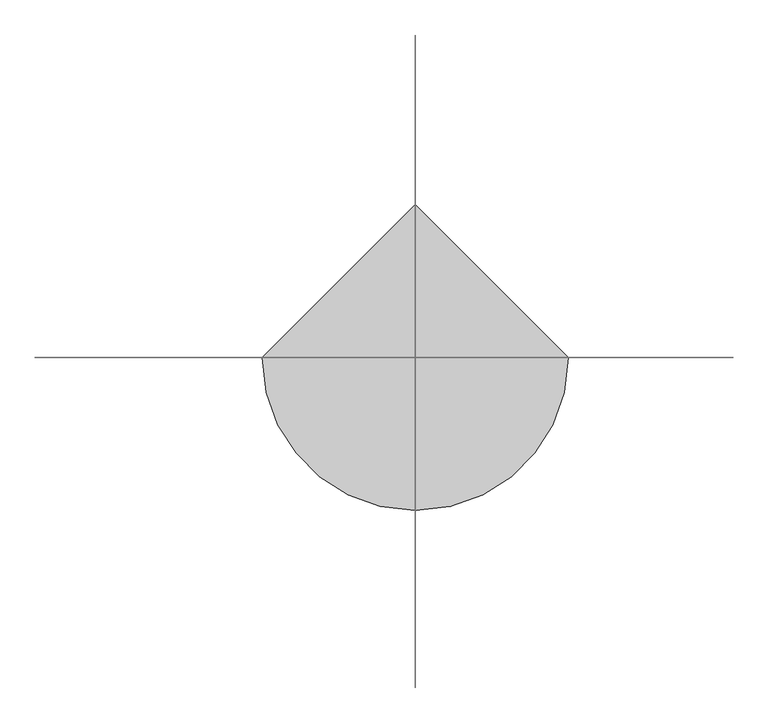
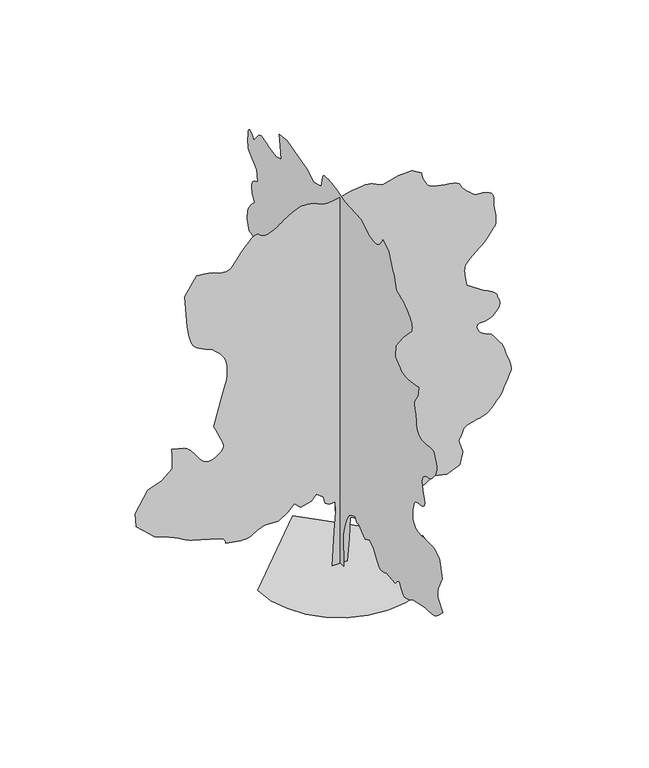
"""IFC4 building model written with IfcOpenShell, lengths in millimetres: geographic element geometry, RPC 木 - 落葉樹 : シュマード オーク - 9.1 メートル."""

from ifc_helpers import new_model, si_unit, origin, place, context, project, spatial, triangles, source, transform, mapped, element, save


def geographic_element_5c09a096(model_context):
    return source(origin(), model_context, "Body", "Tessellation", [
        triangles([(-0.0016876, 163.832478, 0.0085608), (-0.0016876, -150.8808976, 0.0085608), (-0.0016876, -123.5141451, 779.9515205), (-0.0016876, -178.2471505, 1012.5653744), (-0.0016876, -260.3461545, 1231.4963425), (-0.0016876, -356.128771, 1382.0105564), (-0.0016876, -465.5942914, 1450.4274559), (-0.0016876, -602.4255469, 1505.1588535), (-0.0016876, -657.1595243, 1382.0105564), (-0.0016876, -752.9421953, 1409.3763279), (-0.0016876, -862.4076794, 1299.9107712), (-0.0016876, -1012.9218206, 1204.1281002), (-0.0016876, -1190.8042042, 1286.2278854), (-0.0016876, -1355.0011585, 1176.7624014), (-0.0016876, -1464.4667152, 985.1971321), (-0.0016876, -1490.95536, 947.379019), (-0.0016876, -1518.0429508, 911.3556364), (-0.0016876, -1546.3262535, 878.9241858), (-0.0016876, -1576.4068302, 851.8769268), (-0.0016876, -1608.8788307, 832.0111336), (-0.0016876, -1644.3435265, 821.1189205), (-0.0016876, -1683.3976833, 821.0001051), (-0.0016876, -1720.8568794, 827.6608177), (-0.0016876, -1751.8549873, 835.7598146), (-0.0016876, -1777.4640347, 845.0544508), (-0.0016876, -1798.7681122, 855.307168), (-0.0016876, -1816.8392475, 866.2777193), (-0.0016876, -1832.7565899, 877.7285465), (-0.0016876, -1847.5972538, 889.4144611), (-0.0016876, -2203.3595501, 848.3658766), (-0.0016876, -2238.4248516, 888.8583904), (-0.0016876, -2272.772319, 925.9965305), (-0.0016876, -2305.6839729, 956.4360243), (-0.0016876, -2336.4419792, 976.8200272), (-0.0016876, -2364.326033, 983.8017958), (-0.0016876, -2388.6204803, 974.0293545), (-0.0016876, -2408.6076324, 944.1484749), (-0.0016876, -2428.6731228, 901.1838009), (-0.0016876, -2453.5264023, 856.783386), (-0.0016876, -2482.9269333, 814.5366188), (-0.0016876, -2516.6373756, 778.0354311), (-0.0016876, -2554.4225693, 750.8694294), (-0.0016876, -2596.0299133, 736.6279295), (-0.0016876, -2641.2265732, 738.9003925), (-0.0016876, -2686.5496788, 752.2242886), (-0.0016876, -2728.9909836, 768.4198116), (-0.0016876, -2769.0309814, 787.0116274), (-0.0016876, -2807.1751648, 807.5169165), (-0.0016876, -2843.8787384, 829.4580917), (-0.0016876, -2879.6216148, 852.3547319), (-0.0016876, -2914.8839973, 875.7316481), (-0.0016876, -3407.4725349, 971.5142464), (-0.0016876, -3468.9228539, 971.6356052), (-0.0016876, -3529.5136322, 972.4722548), (-0.0016876, -3588.4361984, 974.7472612), (-0.0016876, -3644.831012, 979.1734446), (-0.0016876, -3697.8891106, 986.4761965), (-0.0016876, -3746.7762428, 997.3658661), (-0.0016876, -3790.6081604, 1012.5653744), (-0.0016876, -3832.8471519, 1034.5444107), (-0.0016876, -3877.2604294, 1064.4252903), (-0.0016876, -3923.4427849, 1100.8885443), (-0.0016876, -3971.0916206, 1142.6146311), (-0.0016876, -4019.8017288, 1188.2915668), (-0.0016876, -4069.2199333, 1236.6025715), (-0.0016876, -4119.0171844, 1286.2278854), (-0.0016876, -3927.4367271, 1505.1588535), (-0.0016876, -3921.7492836, 1546.169577), (-0.0016876, -3916.9969574, 1586.9401989), (-0.0016876, -3914.1660255, 1627.2304722), (-0.0016876, -3914.1913147, 1666.8053822), (-0.0016876, -3918.0588112, 1705.4197403), (-0.0016876, -3926.7289215, 1742.8410027), (-0.0016876, -3941.1373444, 1778.8239807), (-0.0016876, -4091.6412392, 2093.5376198), (-0.0016876, -3995.8636551, 2476.6656876), (-0.0016876, -3988.3562645, 2487.2368446), (-0.0016876, -3966.0105354, 2514.3244354), (-0.0016876, -3929.0799408, 2550.9846977), (-0.0016876, -3877.7659218, 2590.2918915), (-0.0016876, -3812.3469498, 2625.276384), (-0.0016876, -3733.0506271, 2649.0121445), (-0.0016876, -3640.1039749, 2654.5478531), (-0.0016876, -3536.5408195, 2650.2507317), (-0.0016876, -3429.8685516, 2648.5572304), (-0.0016876, -3327.0132019, 2648.8098312), (-0.0016876, -3234.9513794, 2650.2507317), (-0.0016876, -3160.5841164, 2652.1465462), (-0.0016876, -3110.8880219, 2653.8400475), (-0.0016876, -3092.7638374, 2654.5478531), (-0.0016876, -3082.1470436, 2661.7773537), (-0.0016876, -3054.7966782, 2682.1514008), (-0.0016876, -3017.3603004, 2713.7991783), (-0.0016876, -2976.5872078, 2754.7490044), (-0.0016876, -2939.1758286, 2803.1562241), (-0.0016876, -2911.8254631, 2857.0482834), (-0.0016876, -2901.2086693, 2914.5302399), (-0.0016876, -2903.2056404, 2971.9613274), (-0.0016876, -2908.7919273, 3027.268998), (-0.0016876, -2917.3611717, 3080.7570122), (-0.0016876, -2928.331723, 3132.8291245), (-0.0016876, -2941.0969322, 3183.8143845), (-0.0016876, -2955.050441, 3234.0668404), (-0.0016876, -2969.6103081, 3283.9652481), (-0.0016876, -2981.5921349, 3298.5756935), (-0.0016876, -2994.9892822, 3312.8070923), (-0.0016876, -3011.2682304, 3326.3306854), (-0.0016876, -3031.8443001, 3338.7927155), (-0.0016876, -3058.1839714, 3349.7885559), (-0.0016876, -3091.7022743, 3359.0150276), (-0.0016876, -3133.8151108, 3366.0675041), (-0.0016876, -3184.7497925, 3370.3899147), (-0.0016876, -3239.7795731, 3375.4201309), (-0.0016876, -3292.8629608, 3386.8964653), (-0.0016876, -3338.0596207, 3410.5816475), (-0.0016876, -3369.3789299, 3452.2395699), (-0.0016876, -3380.8296844, 3517.5826744), (-0.0016876, -3366.4212616, 3612.3742722), (-0.0016876, -3336.9474792, 3719.5267433), (-0.0016876, -3309.8750038, 3817.8070816), (-0.0016876, -3289.2480652, 3906.78479), (-0.0016876, -3279.1370544, 3985.9296684), (-0.0016876, -3283.6617783, 4054.7862213), (-0.0016876, -3306.841468, 4112.8745361), (-0.0016876, -3352.7459335, 4159.6891205), (-0.0016876, -3409.0395905, 4192.4996178), (-0.0016876, -3461.2637283, 4212.5954842), (-0.0016876, -3510.3531738, 4225.7653198), (-0.0016876, -3557.3192024, 4237.7218575), (-0.0016876, -3603.071933, 4254.2534065), (-0.0016876, -3648.5973518, 4281.0479919), (-0.0016876, -3694.8305763, 4323.8936325), (-0.0016876, -3741.9483398, 4378.3926315), (-0.0016876, -3786.8921082, 4436.4809464), (-0.0016876, -3825.8705429, 4498.38647), (-0.0016876, -3855.0411461, 4564.3615128), (-0.0016876, -3870.5617104, 4634.6589661), (-0.0016876, -3868.5900284, 4709.5064323), (-0.0016876, -3845.3344711, 4789.131514), (-0.0016876, -3817.2507202, 4864.434185), (-0.0016876, -3798.2672859, 4925.8842133), (-0.0016876, -3780.7244614, 4972.9516891), (-0.0016876, -3756.9381226, 5005.1811172), (-0.0016876, -3719.2741425, 5022.091713), (-0.0016876, -3660.0733955, 5023.2038544), (-0.0016876, -3571.677047, 5008.0623367), (-0.0016876, -3466.799437, 4991.303476), (-0.0016876, -3365.9916367, 4987.9414719), (-0.0016876, -3273.3231651, 4998.0019043), (-0.0016876, -3192.8638321, 5021.4597748), (-0.0016876, -3128.6584488, 5058.3150833), (-0.0016876, -3084.8265312, 5108.592247), (-0.0016876, -3065.3878922, 5172.2418503), (-0.0016876, -3058.7400421, 5240.239444), (-0.0016876, -3050.651001, 5303.8884659), (-0.0016876, -3041.3489525, 5363.9737518), (-0.0016876, -3031.0859161, 5421.1778183), (-0.0016876, -3020.1153648, 5476.2325974), (-0.0016876, -3008.6646103, 5529.8467667), (-0.0016876, -2996.9862534, 5582.753421), (-0.0016876, -2985.6113663, 5620.8976044), (-0.0016876, -2976.4101837, 5659.1429443), (-0.0016876, -2971.4811241, 5697.6411758), (-0.0016876, -2973.0481796, 5736.4928741), (-0.0016876, -2983.2097687, 5775.8253571), (-0.0016876, -3004.1651756, 5815.7641983), (-0.0016876, -3038.0375267, 5856.4105545), (-0.0016876, -3074.2606064, 5906.2836731), (-0.0016876, -3101.6109718, 5968.8211349), (-0.0016876, -3121.3277916, 6036.6414139), (-0.0016876, -3134.573204, 6102.3129868), (-0.0016876, -3142.5610886, 6158.4049118), (-0.0016876, -3146.4538742, 6197.4839218), (-0.0016876, -3147.4904388, 6212.1702347), (-0.0016876, -3127.318705, 6207.6710907), (-0.0016876, -3073.1481743, 6196.2200455), (-0.0016876, -2994.5596573, 6180.9523727), (-0.0016876, -2901.1328018, 6164.9516052), (-0.0016876, -2802.4231293, 6151.3518539), (-0.0016876, -2708.0358673, 6143.2378143), (-0.0016876, -2627.525956, 6143.7685959), (-0.0016876, -2559.5539421, 6155.5986877), (-0.0016876, -2495.8918396, 6178.2223068), (-0.0016876, -2435.8141113, 6209.8197968), (-0.0016876, -2378.6078648, 6248.5959183), (-0.0016876, -2323.5554111, 6292.7560135), (-0.0016876, -2269.9412418, 6340.5060059), (-0.0016876, -2217.0422905, 6390.0506561), (-0.0016876, -2230.7251762, 6677.4081161), (-0.0016876, -2531.7483719, 7060.5440323), (-0.0016876, -2873.832724, 7416.3037125), (-0.0016876, -2879.1916992, 7460.4132294), (-0.0016876, -2881.4162727, 7505.3825775), (-0.0016876, -2877.4223305, 7552.0204285), (-0.0016876, -2864.1007599, 7601.1604523), (-0.0016876, -2838.3427391, 7653.6624802), (-0.0016876, -2797.0135757, 7710.3351837), (-0.0016876, -2737.0041573, 7772.0633926), (-0.0016876, -2666.6308365, 7831.3905853), (-0.0016876, -2596.257225, 7881.3648605), (-0.0016876, -2525.8914619, 7923.5785629), (-0.0016876, -2455.5207573, 7959.5490417), (-0.0016876, -2385.149762, 7990.8680603), (-0.0016876, -2314.778912, 8019.0779663), (-0.0016876, -2244.408062, 8045.7211075), (-0.0016876, -2223.8648392, 8115.8918243), (-0.0016876, -2203.2002575, 8184.8754044), (-0.0016876, -2182.2954288, 8251.4568054), (-0.0016876, -2161.0317558, 8314.4488907), (-0.0016876, -2139.2903503, 8372.6383621), (-0.0016876, -2116.9523243, 8424.8625), (-0.0016876, -2093.8939934, 8469.9074249), (-0.0016876, -2068.3230251, 8519.0224503), (-0.0016876, -2040.1180607, 8579.6135193), (-0.0016876, -2011.6754654, 8644.7543106), (-0.0016876, -1985.3865177, 8707.4935043), (-0.0016876, -1963.6451122, 8760.9309402), (-0.0016876, -1948.8448528, 8798.0641388), (-0.0016876, -1943.3773087, 8811.991777), (-0.0016876, -1710.7634548, 8948.8206345), (-0.0016876, -1698.8374386, 8925.2366089), (-0.0016876, -1685.7130943, 8900.944487), (-0.0016876, -1670.1925301, 8875.2117554), (-0.0016876, -1651.0851208, 8847.3303177), (-0.0016876, -1627.1900677, 8816.5670792), (-0.0016876, -1597.3090427, 8782.2145248), (-0.0016876, -1560.2493862, 8743.5651398), (-0.0016876, -1515.6087971, 8710.0974152), (-0.0016876, -1464.5071198, 8690.2794388), (-0.0016876, -1408.0188526, 8681.811351), (-0.0016876, -1347.2231449, 8682.4432892), (-0.0016876, -1283.194495, 8689.9003922), (-0.0016876, -1217.0121975, 8701.9072174), (-0.0016876, -1149.7530762, 8716.1894852), (-0.0016876, -848.7223228, 8921.4449799), (-0.0016876, -191.9302724, 8962.4959625), (-0.0016876, -107.0787747, 8985.8276779), (-0.0016876, -23.3040577, 9008.451297), (-0.0016876, 58.316385, 9029.633725), (-0.0016876, 136.7053639, 9048.6680283), (-0.0016876, 210.7859892, 9064.8205307), (-0.0016876, 279.4814509, 9077.3837173), (-0.0016876, 341.7128632, 9085.6494919), (-0.0016876, 403.0696558, 9091.9438751), (-0.0016876, 467.2954957, 9097.530162), (-0.0016876, 530.565798, 9100.0073364), (-0.0016876, 589.0485291, 9096.9738007), (-0.0016876, 638.9140537, 9086.0541183), (-0.0016876, 676.3327726, 9064.8205307), (-0.0016876, 697.4776302, 9030.9231812), (-0.0016876, 765.8919863, 8757.2404678), (-0.0016876, 1066.9227396, 8675.163501), (-0.0016876, 1340.5877941, 8839.3424332), (-0.0016876, 1682.6672047, 8921.4449799), (-0.0016876, 2134.2120266, 9058.2738373), (-0.0016876, 2435.2427799, 9017.2222733), (-0.0016876, 2407.8745377, 8757.2404678), (-0.0016876, 2353.14314, 8456.2320969), (-0.0016876, 2572.0665504, 8387.8054596), (-0.0016876, 2790.9973732, 8428.8564423), (-0.0016876, 2875.6529617, 8460.6556641), (-0.0016876, 2958.0331078, 8489.7004028), (-0.0016876, 3035.8635315, 8513.2338501), (-0.0016876, 3106.8687904, 8528.5015228), (-0.0016876, 3168.7996033, 8532.7733551), (-0.0016876, 3219.3296585, 8523.2692841), (-0.0016876, 3256.2352547, 8497.2580811), (-0.0016876, 3461.49104, 8250.9766022), (-0.0016876, 3508.1286003, 8305.5005997), (-0.0016876, 3553.0726593, 8352.972702), (-0.0016876, 3594.6797127, 8386.33927), (-0.0016876, 3631.2568405, 8398.4978302), (-0.0016876, 3661.1352493, 8382.4209045), (-0.0016876, 3682.6464363, 8331.0315994), (-0.0016876, 3694.0974815, 8237.2762756), (-0.0016876, 3697.5603516, 8133.1570496), (-0.0016876, 3696.7263908, 8052.7480042), (-0.0016876, 3692.302533, 7992.0563599), (-0.0016876, 3684.9974556, 7947.1881683), (-0.0016876, 3675.5433815, 7914.1500687), (-0.0016876, 3664.6486977, 7889.0236954), (-0.0016876, 3653.0462082, 7867.8412674), (-0.0016876, 3338.3378014, 7607.8588806), (-0.0016876, 3310.9618561, 7320.5264191), (-0.0016876, 3354.7176155, 7302.679834), (-0.0016876, 3397.1845001, 7283.418219), (-0.0016876, 3436.9968956, 7261.2748032), (-0.0016876, 3472.8409286, 7234.8345566), (-0.0016876, 3503.4521416, 7202.6307083), (-0.0016876, 3527.4660828, 7163.2476471), (-0.0016876, 3543.5680069, 7115.270343), (-0.0016876, 3549.7359444, 7062.4904251), (-0.0016876, 3545.8178696, 7009.7105072), (-0.0016876, 3533.5328636, 6956.9300079), (-0.0016876, 3514.5491386, 6904.15009), (-0.0016876, 3490.5351974, 6851.3701721), (-0.0016876, 3463.1595428, 6798.5902542), (-0.0016876, 3434.1153854, 6745.8103363), (-0.0016876, 3477.9217232, 6701.8269745), (-0.0016876, 3520.6412086, 6657.6918777), (-0.0016876, 3561.2119881, 6613.3294693), (-0.0016876, 3598.5472092, 6568.6130127), (-0.0016876, 3631.5853088, 6523.4157715), (-0.0016876, 3659.2394348, 6477.6127533), (-0.0016876, 3680.4221535, 6431.1016388), (-0.0016876, 3695.6139587, 6385.7782425), (-0.0016876, 3706.5089333, 6343.3372284), (-0.0016876, 3713.8140106, 6303.2972305), (-0.0016876, 3718.2375778, 6265.1530472), (-0.0016876, 3720.5127296, 6228.4494736), (-0.0016876, 3721.346981, 6192.7068878), (-0.0016876, 3721.4731361, 6157.443924), (-0.0016876, 3639.3708801, 5924.8377731), (-0.0016876, 3601.2772751, 5918.7207047), (-0.0016876, 3563.2848267, 5911.1880249), (-0.0016876, 3525.5449791, 5900.7735443), (-0.0016876, 3488.1591797, 5886.0616516), (-0.0016876, 3451.2788727, 5865.5867386), (-0.0016876, 3414.9546364, 5837.9326126), (-0.0016876, 3379.388784, 5801.6842438), (-0.0016876, 3346.9826225, 5758.63629), (-0.0016876, 3319.6319664, 5711.9990204), (-0.0016876, 3296.4522766, 5662.378212), (-0.0016876, 3276.6093018, 5610.3569687), (-0.0016876, 3259.2940796, 5556.5404861), (-0.0016876, 3243.6723587, 5501.535704), (-0.0016876, 3228.8596001, 5445.9245636), (-0.0016876, 3196.8324852, 5401.9162033), (-0.0016876, 3166.1201157, 5357.806105), (-0.0016876, 3138.0363647, 5313.4436966), (-0.0016876, 3113.8959778, 5268.7022415), (-0.0016876, 3095.0389893, 5223.5050003), (-0.0016876, 3082.7286942, 5177.7269806), (-0.0016876, 3078.3554146, 5131.2158661), (-0.0016876, 3092.0307426, 4761.7558594), (-0.0016876, 3124.0578575, 4758.5203011), (-0.0016876, 3154.7955162, 4753.4897942), (-0.0016876, 3182.8792671, 4744.8955513), (-0.0016876, 3206.9943649, 4730.8914642), (-0.0016876, 3225.8766426, 4709.7087456), (-0.0016876, 3238.1616486, 4679.5271576), (-0.0016876, 3242.5602173, 4638.60233), (-0.0016876, 3241.3466286, 4591.3075424), (-0.0016876, 3238.0102043, 4543.2543709), (-0.0016876, 3232.8535423, 4494.6451286), (-0.0016876, 3226.2812691, 4445.530394), (-0.0016876, 3218.6221436, 4396.0619019), (-0.0016876, 3210.2299232, 4346.3658073), (-0.0016876, 3201.5089439, 4296.5179779), (-0.0016876, 3187.8083267, 4022.8605537), (-0.0016876, 3447.7904228, 4036.5608803), (-0.0016876, 3735.1484642, 4091.2874817), (-0.0016876, 3796.2956039, 4070.5849663), (-0.0016876, 3854.9399895, 4048.7955986), (-0.0016876, 3908.5541588, 4024.8575249), (-0.0016876, 3954.6356483, 3997.6838928), (-0.0016876, 3990.6564148, 3966.2128487), (-0.0016876, 4014.1142853, 3929.3578308), (-0.0016876, 4022.4812164, 3886.0316963), (-0.0016876, 4020.1051987, 3831.1536507), (-0.0016876, 4013.4064796, 3761.8924713), (-0.0016876, 4003.0931557, 3680.6747543), (-0.0016876, 3989.9486092, 3589.8770988), (-0.0016876, 3974.6303581, 3491.9002304), (-0.0016876, 3957.8712067, 3389.1207481), (-0.0016876, 3940.4042496, 3283.9652481), (-0.0016876, 3817.2507202, 2955.5812225), (-0.0016876, 3749.986512, 2917.841375), (-0.0016876, 3683.8094467, 2882.3766792), (-0.0016876, 3619.7807968, 2851.4619965), (-0.0016876, 3558.9877052, 2827.3721878), (-0.0016876, 3502.4917351, 2812.3571159), (-0.0016876, 3451.3800293, 2808.742511), (-0.0016876, 3406.7394402, 2818.7526558), (-0.0016876, 3023.6291039, 2982.9318787), (-0.0016876, 2640.4934784, 2859.8036385), (-0.0016876, 2366.8258804, 2668.2231812), (-0.0016876, 2093.1635147, 2257.7345741), (-0.0016876, 2066.6748699, 2216.9235477), (-0.0016876, 2039.5871338, 2177.5508057), (-0.0016876, 2011.3013603, 2141.0496906), (-0.0016876, 1981.2232544, 2108.8558708), (-0.0016876, 1948.7513992, 2082.4077759), (-0.0016876, 1913.2867035, 2063.1384579), (-0.0016876, 1874.2324013, 2052.4864918), (-0.0016876, 1835.2565826, 2048.9374352), (-0.0016876, 1798.6745132, 2049.2154705), (-0.0016876, 1761.8523422, 2052.1275021), (-0.0016876, 1722.1611603, 2056.4752018), (-0.0016876, 1676.9620296, 2061.0631485), (-0.0016876, 1623.6258957, 2064.6930141), (-0.0016876, 1559.5187622, 2066.1692322), (-0.0016876, 1490.7430183, 2060.9848103), (-0.0016876, 1424.841227, 2046.4627316), (-0.0016876, 1361.330714, 2024.1626392), (-0.0016876, 1299.7363632, 1995.6392349), (-0.0016876, 1239.5776806, 1962.4494003), (-0.0016876, 1180.377079, 1926.1479824), (-0.0016876, 1121.6567533, 1888.2893921), (-0.0016876, 1039.5570408, 1655.6755383), (-0.0016876, 806.9431143, 1395.6934422), (-0.0016876, 774.8277054, 1360.9060307), (-0.0016876, 737.6895653, 1326.8392147), (-0.0016876, 696.3603292, 1293.368874), (-0.0016876, 651.6793356, 1260.3788818), (-0.0016876, 604.4856683, 1227.745118), (-0.0016876, 555.6186293, 1195.3542171), (-0.0016876, 505.912361, 1163.0795156), (-0.0016876, 423.8126121, 1450.4274559), (-0.0016876, 286.9813747, 1641.9901817), (-0.0016876, 232.2486145, 1518.8417393), (-0.0016876, 191.1987401, 1327.2790134), (-0.0016876, 177.5158725, 985.1971321), (-0.0016876, 150.1493652, 506.2865024), (169.54274, 0.0004339, 0.0216695), (-186.21952, 0.0004339, 0.0216695), (-131.4872685, 0.0003851, 821.0127497), (-104.1207703, 0.0003564, 1299.9234158), (-117.8038922, 0.0003417, 1546.2226261), (-254.6358926, 0.0003425, 1532.5397404), (-350.4185454, 0.0003394, 1587.2712833), (-391.46713, 0.0003287, 1765.1537395), (-555.6666641, 0.0003221, 1874.6191509), (-665.1321482, 0.0003294, 1751.4708538), (-911.4288877, 0.0003336, 1683.0539543), (-1061.9455725, 0.0003255, 1819.8851372), (-1212.4597137, 0.0003344, 1669.3710686), (-1431.3906818, 0.0003425, 1532.5397404), (-1759.7872066, 0.0003417, 1546.2226261), (-1923.984161, 0.0003459, 1477.8057266), (-1959.2517757, 0.0003475, 1451.5952625), (-1994.9946522, 0.000349, 1426.464093), (-2031.6954643, 0.0003503, 1403.4865711), (-2069.8345608, 0.0003514, 1383.7395206), (-2109.8872032, 0.0003524, 1368.2999107), (-2152.3311241, 0.000353, 1358.2468906), (-2197.6492882, 0.0003532, 1354.6574295), (-2248.1541996, 0.0003532, 1356.2523903), (-2305.1203445, 0.000353, 1360.7215942), (-2367.4704632, 0.0003524, 1367.5819313), (-2434.1331093, 0.0003519, 1376.3584305), (-2504.0236107, 0.0003514, 1386.5705978), (-2576.0604927, 0.0003506, 1397.7408463), (-2649.1891685, 0.0003501, 1409.3914433), (-2652.5761711, 0.0003483, 1438.632827), (-2658.7188194, 0.0003464, 1467.3938622), (-2670.3718872, 0.0003449, 1495.1994324), (-2690.2907295, 0.0003433, 1521.5691891), (-2721.2054123, 0.0003417, 1546.022929), (-2765.8712906, 0.0003404, 1568.0829197), (-2827.0690086, 0.0003394, 1587.2712833), (-3429.1354568, 0.0003287, 1765.1537395), (-3478.2754807, 0.0003279, 1780.7500259), (-3530.7775085, 0.0003266, 1802.8124874), (-3584.9477486, 0.000325, 1829.4200203), (-3639.1182793, 0.0003232, 1858.6612587), (-3691.6203072, 0.0003213, 1888.6206219), (-3740.7856201, 0.0003198, 1917.3841278), (-3784.895137, 0.0003182, 1943.0335796), (-3832.3416595, 0.0003166, 1967.6870167), (-3891.2642258, 0.0003151, 1994.4965721), (-3959.741732, 0.0003132, 2023.09846), (-4035.903653, 0.0003117, 2053.1386322), (-4117.8038864, 0.0003098, 2084.2556282), (-4203.5207474, 0.0003078, 2116.0878422), (-4291.1842918, 0.0003059, 2148.281662), (-4715.3456108, 0.0002822, 2545.0952316), (-4742.7215561, 0.0002626, 2873.4789665), (-4455.3635147, 0.0002349, 3338.716848), (-4126.9797798, 0.0002276, 3461.8703773), (-3880.6727211, 0.0002153, 3667.125872), (-3880.6727211, 0.0001967, 3981.8345695), (-3894.3733383, 0.0001868, 4146.0390816), (-3607.0152969, 0.000191, 4077.6121536), (-3574.6597137, 0.0001923, 4056.7579033), (-3541.7227707, 0.0001936, 4033.8563942), (-3507.5725296, 0.0001952, 4006.8847847), (-3471.6276306, 0.000197, 3973.8213959), (-3433.281134, 0.0001996, 3932.5933891), (-3391.9519707, 0.0002027, 3881.2290825), (-3347.0332008, 0.0002064, 3817.6300575), (-3301.507782, 0.0002103, 3750.8207634), (-3257.6761551, 0.000214, 3691.8981972), (-3213.8445282, 0.0002168, 3642.0756569), (-3168.3191093, 0.0002192, 3602.5411514), (-3119.4572662, 0.000221, 3574.4829803), (-3065.5649162, 0.0002218, 3559.1391495), (-3004.9488487, 0.0002218, 3557.6479614), (-2938.6956253, 0.000221, 3572.8144775), (-2871.9621986, 0.0002192, 3603.5271378), (-2809.2732925, 0.0002166, 3645.2606369), (-2755.2294983, 0.0002137, 3693.4402542), (-2714.3299599, 0.0002108, 3743.5406845), (-2691.1502701, 0.000208, 3791.0124962), (-2690.2401512, 0.0002056, 3831.3053856), (-2706.3673645, 0.000203, 3874.8841209), (-2730.3813057, 0.0001996, 3933.5287971), (-2760.9675201, 0.0001952, 4004.7363693), (-2796.8365517, 0.0001905, 4085.9790848), (-2836.6492378, 0.0001852, 4174.7800598), (-2879.0905426, 0.0001795, 4268.6112511), (-2922.8465927, 0.0001737, 4364.970195), (-2731.2914246, 0.0001322, 5062.7892288), (-2705.078199, 0.0001275, 5141.7820816), (-2679.9521164, 0.0001228, 5219.6883728), (-2656.9747398, 0.0001183, 5295.4459579), (-2637.2326309, 0.0001139, 5367.9932739), (-2621.7879341, 0.00011, 5436.1925995), (-2611.7275017, 0.0001061, 5499.0335312), (-2608.1378952, 0.0001029, 5555.4027649), (-2609.0733032, 9.95e-05, 5610.407547), (-2612.1318375, 9.61e-05, 5668.7737518), (-2617.8445702, 9.25e-05, 5728.8084595), (-2626.6664154, 8.88e-05, 5788.8431671), (-2639.052578, 8.54e-05, 5847.2099533), (-2655.5338394, 8.2e-05, 5902.2141541), (-2676.5648232, 7.92e-05, 5952.2134277), (-2703.6123001, 7.63e-05, 5998.7245422), (-2737.130603, 7.37e-05, 6044.5281418), (-2776.0078812, 7.11e-05, 6089.7248016), (-2819.2075699, 6.82e-05, 6134.4412582), (-2865.6428169, 6.56e-05, 6178.8036667), (-2914.2520592, 6.3e-05, 6222.913765), (-2963.8975754, 6.03e-05, 6266.9221252), (-3042.7389839, 5.85e-05, 6299.2271301), (-3119.5331337, 5.64e-05, 6331.9111816), (-3192.2571831, 5.46e-05, 6365.3033295), (-3258.864164, 5.25e-05, 6399.7570404), (-3317.3571053, 5.04e-05, 6435.6769409), (-3365.6628777, 4.81e-05, 6473.3659195), (-3401.7598022, 4.57e-05, 6513.229184), (-3430.1720215, 4.26e-05, 6566.36315), (-3456.4355347, 3.84e-05, 6638.4046829), (-3480.0451401, 3.34e-05, 6721.4676361), (-3500.5453423, 2.82e-05, 6807.6397018), (-3517.4562286, 2.33e-05, 6889.0085724), (-3530.2973053, 1.93e-05, 6957.713681), (-3538.6136581, 1.65e-05, 7005.8177216), (-3593.3399689, -2.93e-05, 7772.0633926), (-3319.6572556, -5.46e-05, 8196.2502914), (-3246.5538689, -5.41e-05, 8187.3525787), (-3174.512336, -5.36e-05, 8177.8729248), (-3104.6192184, -5.28e-05, 8167.1805542), (-3037.9363701, -5.2e-05, 8154.6935257), (-2975.6012215, -5.12e-05, 8139.8048996), (-2918.6250481, -5.02e-05, 8121.933316), (-2868.1199913, -4.89e-05, 8100.4724167), (-2816.7809738, -4.75e-05, 8079.7196136), (-2758.970549, -4.68e-05, 8065.2100342), (-2698.3039032, -4.62e-05, 8058.1069794), (-2638.3447723, -4.65e-05, 8059.6237473), (-2582.6830536, -4.7e-05, 8070.948056), (-2534.9333519, -4.83e-05, 8093.2937851), (-2498.6774254, -5.04e-05, 8127.8230728), (-2279.7464573, -6.77e-05, 8415.1811142), (-2221.2636898, -7.16e-05, 8482.1165634), (-2163.7390034, -7.55e-05, 8546.0696365), (-2108.130479, -7.89e-05, 8604.0317963), (-2055.3908203, -8.18e-05, 8653.0200851), (-2006.4833405, -8.41e-05, 8690.0521271), (-1962.3608883, -8.54e-05, 8712.0943863), (-1923.984161, -8.57e-05, 8716.2144836), (-1893.107412, -8.49e-05, 8705.9261581), (-1867.9762424, -8.39e-05, 8689.1672974), (-1844.2807411, -8.28e-05, 8669.5266357), (-1817.7112873, -8.18e-05, 8650.6184875), (-1783.9629112, -8.07e-05, 8636.0333313), (-1738.7232307, -8.05e-05, 8629.334903), (-1677.6874214, -8.07e-05, 8634.111937), (-1604.7635296, -8.2e-05, 8654.8653214), (-1529.9260918, -8.39e-05, 8689.4957657), (-1457.9576649, -8.65e-05, 8731.7600464), (-1393.6509796, -8.91e-05, 8775.491098), (-1341.7910637, -9.14e-05, 8814.4189545), (-1307.1629448, -9.3e-05, 8842.3509705), (-1294.5568829, -9.38e-05, 8853.0433411), (-1279.1197437, -9.43e-05, 8862.9270401), (-1238.0710865, -9.59e-05, 8888.6341919), (-1179.3078856, -9.8e-05, 8924.1244675), (-1110.7316935, -0.0001003, 8963.456369), (-1040.242028, -0.0001024, 9000.6401459), (-975.7356457, -0.0001042, 9029.6843033), (-925.1117735, -0.000105, 9044.5985092), (-877.0814203, -0.0001053, 9047.909935), (-817.3222046, -0.0001053, 9045.9635422), (-749.1858839, -0.0001048, 9038.5064392), (-676.0218178, -0.000104, 9025.3113144), (-601.18438, -0.0001029, 9006.1252762), (-528.0203502, -0.0001014, 8980.6960144), (-459.8840295, -9.95e-05, 8948.8206345), (-387.3999364, -9.8e-05, 8922.8100128), (-300.5530209, -9.74e-05, 8913.3309402), (-201.738322, -9.74e-05, 8917.6027725), (-93.349898, -9.85e-05, 8932.8704453), (22.2192106, -9.98e-05, 8956.4038925), (142.5753726, -0.0001016, 8985.4480499), (265.3258833, -0.0001035, 9017.2478531), (350.0570486, -0.0001042, 9028.7238968), (432.9935197, -0.0001048, 9038.7843292), (512.3405296, -0.0001053, 9045.9635422), (586.3008408, -0.0001053, 9048.8447617), (653.0822296, -0.0001053, 9045.9635422), (710.8874949, -0.0001045, 9035.9025284), (757.9193624, -0.0001035, 9017.2478531), (797.3729862, -0.0001022, 8995.3823273), (833.9549829, -0.0001011, 8976.3986023), (868.1432304, -0.0001001, 8959.7914764), (900.4153885, -9.93e-05, 8945.1051636), (931.2542765, -9.85e-05, 8931.8844589), (961.1326853, -9.77e-05, 8919.5741638), (990.533289, -9.69e-05, 8907.7696518), (1346.2955853, -0.0001027, 9003.5469452), (1661.0092243, -0.0001035, 9017.2478531), (1879.9426632, -9.61e-05, 8894.0943237), (1883.0923256, -9.43e-05, 8861.7137421), (1887.5613842, -9.22e-05, 8828.4733292), (1894.6619682, -9.01e-05, 8793.5644135), (1905.7134739, -8.8e-05, 8756.1533249), (1922.0277397, -8.54e-05, 8715.3802322), (1944.9269234, -8.28e-05, 8670.4108841), (1975.7228634, -7.99e-05, 8620.4366089), (2006.6805668, -7.71e-05, 8574.684169), (2032.3702778, -7.52e-05, 8540.8873947), (2057.5824017, -7.37e-05, 8515.963916), (2087.1042915, -7.24e-05, 8496.7528793), (2125.718795, -7.16e-05, 8480.1957504), (2178.2182068, -7.05e-05, 8463.1839981), (2249.3878452, -6.92e-05, 8442.5567688), (2337.1118511, -6.82e-05, 8422.6887955), (2431.7772938, -6.71e-05, 8407.5978561), (2526.9204689, -6.64e-05, 8393.7202148), (2616.0752014, -6.53e-05, 8377.4415573), (2692.7931931, -6.4e-05, 8355.171405), (2750.6036179, -6.22e-05, 8323.3471848), (2783.0350685, -5.96e-05, 8278.3522568), (2806.9984314, -5.64e-05, 8225.9769653), (2842.4631271, -5.33e-05, 8174.3091888), (2887.5080521, -5.02e-05, 8123.2477707), (2940.2123932, -4.73e-05, 8072.6671371), (2998.6547562, -4.42e-05, 8022.4399704), (3060.9137466, -4.13e-05, 7972.4656952), (3125.1194206, -3.81e-05, 7922.5925766), (3215.3865852, -3.76e-05, 7913.3408157), (3301.9629868, -3.71e-05, 7901.3339905), (3381.1075745, -3.61e-05, 7883.8164551), (3449.1301666, -3.45e-05, 7858.0331451), (3502.2894218, -3.21e-05, 7821.2539948), (3536.9201569, -2.93e-05, 7770.7239395), (3549.2810303, -2.53e-05, 7703.6617538), (3550.0897018, -2.12e-05, 7633.7939255), (3552.3142754, -1.75e-05, 7575.4527191), (3555.7521469, -1.46e-05, 7526.6411636), (3560.150425, -1.23e-05, 7485.5146042), (3565.2565086, -1.02e-05, 7450.1504837), (3570.8427956, -8.1e-06, 7418.5785736), (3576.6566849, -6.5e-06, 7388.9530563), (3588.1077301, -2.4e-06, 7318.807338), (3597.8899818, 1.8e-06, 7250.1272278), (3604.3105202, 5.7e-06, 7184.30392), (3605.7008423, 9.4e-06, 7122.7780243), (3600.3927361, 1.28e-05, 7067.0151489), (3586.717408, 1.57e-05, 7018.4309052), (3562.9813568, 1.8e-05, 6978.4414856), (3532.6986122, 2.04e-05, 6940.1205688), (3500.0145607, 2.3e-05, 6896.2633621), (3464.2463951, 2.59e-05, 6848.1093246), (3424.6360222, 2.87e-05, 6796.8461746), (3380.4756363, 3.19e-05, 6743.6866287), (3331.0324333, 3.53e-05, 6689.7945694), (3275.6233154, 3.84e-05, 6636.3571335), (3211.2914864, 4.18e-05, 6581.2767746), (3139.5025543, 4.52e-05, 6522.3542084), (3066.298011, 4.89e-05, 6460.8027328), (2997.6434807, 5.25e-05, 6397.8106476), (2939.5298767, 5.64e-05, 6334.5906693), (2897.9225327, 6.01e-05, 6272.3066803), (2878.8126526, 6.37e-05, 6212.1958145), (2875.7538277, 6.71e-05, 6152.7424667), (2877.7002205, 7.08e-05, 6091.8735077), (2883.8428688, 7.45e-05, 6029.7912506), (2893.3472305, 7.84e-05, 5966.7735855), (2905.3543465, 8.2e-05, 5903.0228256), (2919.0296745, 8.6e-05, 5838.7924438), (2933.5389633, 8.99e-05, 5774.3335876), (3344.0505341, 0.0001061, 5500.6508743), (3359.950145, 0.0001066, 5493.5733994), (3401.0014183, 0.0001076, 5474.0083145), (3457.1433403, 0.0001095, 5444.6606873), (3518.2901894, 0.0001116, 5408.1088486), (3574.432402, 0.0001142, 5367.0328674), (3615.4833847, 0.0001165, 5324.0099121), (3631.3832863, 0.0001191, 5281.7200516), (3639.9269508, 0.0001215, 5241.8062088), (3659.4667465, 0.0001238, 5201.8673676), (3680.9276459, 0.0001264, 5158.5921021), (3695.209623, 0.0001296, 5108.592247), (3693.2126518, 0.000133, 5048.5575394), (3665.8619957, 0.0001374, 4975.1253937), (3604.0326302, 0.0001429, 4884.9093887), (3518.7453941, 0.0001473, 4808.1658173), (3431.0565605, 0.0001497, 4768.504866), (3346.9573334, 0.0001507, 4752.8072777), (3272.4383354, 0.000151, 4747.8529289), (3213.4654816, 0.0001515, 4740.4969826), (3176.0541023, 0.0001528, 4717.6207626), (3166.170694, 0.000156, 4665.9782753), (3180.4020927, 0.0001596, 4601.5955772), (3209.7241402, 0.0001628, 4547.9814079), (3251.6096649, 0.0001656, 4503.3408188), (3303.5553314, 0.0001677, 4465.8791519), (3363.0339684, 0.0001696, 4433.8014587), (3427.5431122, 0.0001714, 4405.3386612), (3494.5544289, 0.000173, 4378.6455231), (3561.5407471, 0.0001779, 4293.9143578), (3625.7714195, 0.0001829, 4210.9778503), (3684.4919632, 0.0001876, 4131.6309494), (3734.9464417, 0.000192, 4057.6680222), (3774.4050797, 0.0001962, 3990.8840172), (3800.087233, 0.0001996, 3933.0735924), (3809.2631264, 0.0002022, 3886.0569855), (3820.4357002, 0.0002056, 3829.7886177), (3848.3677162, 0.0002106, 3749.379863), (3884.6666634, 0.0002161, 3654.108062), (3920.9656105, 0.0002221, 3553.3505493), (3948.8976265, 0.0002278, 3456.4102455), (3960.070491, 0.000233, 3372.6397774), (3946.0916931, 0.0002367, 3311.3409027), (3913.6602425, 0.0002401, 3250.8259918), (3875.9712639, 0.0002451, 3169.026915), (3834.4397873, 0.0002508, 3074.7408096), (3790.5322929, 0.0002566, 2976.890387), (3745.6388123, 0.000262, 2884.2977829), (3701.2511147, 0.0002667, 2805.8357117), (3658.7589409, 0.0002701, 2750.3507263), (3617.5562233, 0.0002727, 2706.3926537), (3575.3928085, 0.0002756, 2658.3394821), (3531.3082901, 0.0002785, 2608.87099), (3484.3422615, 0.0002814, 2560.6157959), (3433.559024, 0.000284, 2516.1722878), (3377.9984619, 0.0002863, 2478.1949547), (3316.6745888, 0.0002879, 2449.3124153), (3244.2031403, 0.0002892, 2427.889595), (3160.685273, 0.0002905, 2408.6227478), (3073.6033791, 0.0002916, 2388.6355957), (2990.3634018, 0.0002929, 2365.0589825), (2918.3471581, 0.0002947, 2335.0214264), (2865.0108788, 0.000297, 2295.6462135), (2837.7613792, 0.0003002, 2244.064333), (2823.176223, 0.0003033, 2192.3637096), (2804.7232796, 0.0003057, 2152.1517746), (2785.3352188, 0.0003075, 2119.8390667), (2767.8682617, 0.0003093, 2091.8337994), (2755.17892, 0.0003109, 2064.5465115), (2750.1487038, 0.0003127, 2034.3874512), (2755.6591232, 0.0003148, 1997.7675934), (2837.7613792, 0.0003305, 1737.7879681), (2769.3597404, 0.0003483, 1436.7572147), (2468.3188133, 0.0003556, 1313.6087723), (2167.28806, 0.0003516, 1382.023201), (1866.2573067, 0.0003629, 1190.4604025), (1647.3263386, 0.0003556, 1313.6087723), (1332.6126995, 0.0003475, 1450.4401005), (1311.9885223, 0.0003483, 1438.4305138), (1290.7652538, 0.000349, 1424.747628), (1268.3464188, 0.0003501, 1407.7155281), (1244.1303097, 0.0003514, 1385.6530666), (1217.5228495, 0.000353, 1356.8920315), (1187.9225487, 0.0003553, 1319.7512753), (1154.7327868, 0.0003582, 1272.5576443), (1119.9454479, 0.0003611, 1222.9702641), (1085.8785593, 0.0003637, 1179.1283907), (1052.4082912, 0.000366, 1140.0741611), (1019.415683, 0.0003681, 1104.849567), (986.7845352, 0.0003699, 1072.4965273), (954.391091, 0.0003718, 1042.0595043), (922.1189329, 0.0003736, 1012.578019), (963.1675175, 0.0003908, 725.2301514), (939.5909042, 0.0003914, 716.5724676), (915.2964569, 0.0003916, 708.7540495), (889.5661234, 0.0003921, 702.6115465), (861.6796715, 0.0003924, 698.9816809), (830.9242086, 0.0003924, 698.7036455), (796.5767412, 0.0003921, 702.6115465), (757.9193624, 0.0003916, 711.5472656), (717.6670229, 0.0003906, 726.4661951), (678.8529676, 0.0003895, 747.1308495), (641.2345516, 0.000388, 772.5830023), (604.5716369, 0.0003861, 801.8648632), (568.629136, 0.0003843, 834.0182058), (533.1643676, 0.0003822, 868.0850945), (497.9397735, 0.0003801, 903.1125349), (237.9583677, 0.000372, 1039.9437904), (210.5928688, 0.0004021, 533.6648821), (-1907.5334209, 0.0, 0.0), (-1857.1042316, -437.0809155, 0.0), (-1713.4833469, -838.4696056, 0.0), (-1488.1696289, -1192.6646284, 0.0), (-1192.6646284, -1488.1696289, 0.0), (-838.4696056, -1713.4833469, 0.0), (-437.0809155, -1857.1042316, 0.0), (8.34e-05, -1907.5334209, 0.0), (437.0809155, -1857.1042316, 0.0), (838.4696056, -1713.4833469, 0.0), (1192.6646284, -1488.1696289, 0.0), (1488.1696289, -1192.6646284, 0.0), (1713.4833469, -838.4696056, 0.0), (1857.1042316, -437.0809155, 0.0), (1907.5334209, 0.0001667, 0.0), (-0.0002501, 1907.5334209, 0.0)], [[407, 408, 409], [173, 174, 175], [406, 407, 409], [219, 220, 221], [1, 2, 3], [414, 1, 3], [413, 414, 3], [413, 3, 4], [412, 413, 4], [412, 4, 5], [255, 256, 257], [219, 221, 222], [65, 66, 67], [405, 406, 409], [8, 9, 10], [219, 222, 223], [404, 405, 409], [64, 65, 67], [412, 5, 6], [411, 412, 6], [403, 404, 409], [219, 223, 224], [172, 173, 175], [172, 175, 176], [171, 172, 176], [171, 176, 177], [170, 171, 177], [254, 255, 257], [254, 257, 258], [402, 403, 409], [63, 64, 67], [218, 219, 224], [401, 402, 409], [218, 224, 225], [217, 218, 225], [312, 313, 314], [216, 217, 225], [216, 225, 226], [170, 177, 178], [169, 170, 178], [168, 169, 178], [167, 168, 178], [167, 178, 179], [166, 167, 179], [166, 179, 180], [165, 166, 180], [11, 12, 13], [216, 226, 227], [215, 216, 227], [400, 401, 409], [400, 409, 410], [399, 400, 410], [29, 30, 31], [62, 63, 67], [214, 215, 227], [214, 227, 228], [410, 411, 6], [410, 6, 7], [165, 180, 181], [164, 165, 181], [312, 314, 315], [61, 62, 67], [213, 214, 228], [60, 61, 67], [59, 60, 67], [58, 59, 67], [57, 58, 67], [56, 57, 67], [55, 56, 67], [54, 55, 67], [53, 54, 67], [52, 53, 67], [52, 67, 68], [52, 68, 69], [253, 254, 258], [252, 253, 258], [29, 31, 32], [271, 272, 273], [271, 273, 274], [270, 271, 274], [270, 274, 275], [269, 270, 275], [268, 269, 275], [268, 275, 276], [268, 276, 277], [268, 277, 278], [268, 278, 279], [268, 279, 280], [268, 280, 281], [268, 281, 282], [268, 282, 283], [267, 268, 283], [266, 267, 283], [265, 266, 283], [264, 265, 283], [263, 264, 283], [262, 263, 283], [261, 262, 283], [260, 261, 283], [259, 260, 283], [259, 283, 284], [52, 69, 70], [212, 213, 228], [212, 228, 229], [211, 212, 229], [210, 211, 229], [209, 210, 229], [208, 209, 229], [10, 11, 13], [163, 164, 181], [163, 181, 182], [312, 315, 316], [51, 52, 70], [51, 70, 71], [51, 71, 72], [207, 208, 229], [207, 229, 230], [206, 207, 230], [366, 367, 368], [74, 75, 76], [74, 76, 77], [74, 77, 78], [74, 78, 79], [74, 79, 80], [74, 80, 81], [74, 81, 82], [74, 82, 83], [74, 83, 84], [74, 84, 85], [74, 85, 86], [73, 74, 86], [73, 86, 87], [73, 87, 88], [72, 73, 88], [51, 72, 88], [51, 88, 89], [51, 89, 90], [51, 90, 91], [51, 91, 92], [51, 92, 93], [50, 51, 93], [49, 50, 93], [48, 49, 93], [47, 48, 93], [46, 47, 93], [45, 46, 93], [44, 45, 93], [43, 44, 93], [42, 43, 93], [41, 42, 93], [40, 41, 93], [39, 40, 93], [38, 39, 93], [37, 38, 93], [36, 37, 93], [35, 36, 93], [35, 93, 94], [34, 35, 94], [34, 94, 95], [34, 95, 96], [33, 34, 96], [205, 206, 230], [258, 259, 284], [252, 258, 284], [29, 32, 33], [29, 33, 96], [29, 96, 97], [311, 312, 316], [190, 191, 192], [190, 192, 193], [190, 193, 194], [190, 194, 195], [190, 195, 196], [190, 196, 197], [190, 197, 198], [190, 198, 199], [190, 199, 200], [190, 200, 201], [190, 201, 202], [190, 202, 203], [190, 203, 204], [190, 204, 205], [189, 190, 205], [189, 205, 230], [189, 230, 231], [189, 231, 232], [189, 232, 233], [189, 233, 234], [410, 7, 8], [310, 311, 316], [310, 316, 317], [309, 310, 317], [308, 309, 317], [307, 308, 317], [306, 307, 317], [305, 306, 317], [304, 305, 317], [303, 304, 317], [302, 303, 317], [302, 317, 318], [301, 302, 318], [300, 301, 318], [299, 300, 318], [299, 318, 319], [298, 299, 319], [298, 319, 320], [162, 163, 182], [366, 368, 369], [298, 320, 321], [366, 369, 370], [366, 370, 371], [366, 371, 372], [366, 372, 373], [366, 373, 374], [366, 374, 375], [365, 366, 375], [364, 365, 375], [363, 364, 375], [362, 363, 375], [361, 362, 375], [360, 361, 375], [359, 360, 375], [358, 359, 375], [357, 358, 375], [356, 357, 375], [355, 356, 375], [354, 355, 375], [353, 354, 375], [352, 353, 375], [351, 352, 375], [350, 351, 375], [350, 375, 376], [234, 235, 236], [189, 234, 236], [188, 189, 236], [188, 236, 237], [188, 237, 238], [188, 238, 239], [188, 239, 240], [188, 240, 241], [188, 241, 242], [188, 242, 243], [188, 243, 244], [188, 244, 245], [188, 245, 246], [188, 246, 247], [188, 247, 248], [188, 248, 249], [188, 249, 250], [188, 250, 251], [188, 251, 252], [188, 252, 284], [187, 188, 284], [187, 284, 285], [187, 285, 286], [187, 286, 287], [187, 287, 288], [187, 288, 289], [187, 289, 290], [187, 290, 291], [187, 291, 292], [187, 292, 293], [187, 293, 294], [187, 294, 295], [187, 295, 296], [187, 296, 297], [187, 297, 298], [187, 298, 321], [187, 321, 322], [187, 322, 323], [187, 323, 324], [187, 324, 325], [187, 325, 326], [187, 326, 327], [187, 327, 328], [187, 328, 329], [187, 329, 330], [187, 330, 331], [187, 331, 332], [187, 332, 333], [187, 333, 334], [187, 334, 335], [186, 187, 335], [185, 186, 335], [184, 185, 335], [183, 184, 335], [182, 183, 335], [162, 182, 335], [161, 162, 335], [160, 161, 335], [159, 160, 335], [158, 159, 335], [157, 158, 335], [156, 157, 335], [155, 156, 335], [154, 155, 335], [153, 154, 335], [152, 153, 335], [151, 152, 335], [150, 151, 335], [350, 376, 377], [142, 143, 144], [142, 144, 145], [141, 142, 145], [141, 145, 146], [140, 141, 146], [140, 146, 147], [139, 140, 147], [138, 139, 147], [137, 138, 147], [136, 137, 147], [135, 136, 147], [134, 135, 147], [133, 134, 147], [133, 147, 148], [132, 133, 148], [131, 132, 148], [130, 131, 148], [129, 130, 148], [128, 129, 148], [127, 128, 148], [127, 148, 149], [126, 127, 149], [125, 126, 149], [125, 149, 150], [125, 150, 335], [124, 125, 335], [123, 124, 335], [122, 123, 335], [121, 122, 335], [120, 121, 335], [119, 120, 335], [118, 119, 335], [117, 118, 335], [116, 117, 335], [115, 116, 335], [114, 115, 335], [113, 114, 335], [112, 113, 335], [111, 112, 335], [110, 111, 335], [109, 110, 335], [108, 109, 335], [107, 108, 335], [106, 107, 335], [105, 106, 335], [104, 105, 335], [103, 104, 335], [102, 103, 335], [101, 102, 335], [100, 101, 335], [99, 100, 335], [98, 99, 335], [97, 98, 335], [29, 97, 335], [28, 29, 335], [27, 28, 335], [26, 27, 335], [25, 26, 335], [25, 335, 336], [25, 336, 337], [25, 337, 338], [349, 350, 377], [339, 340, 341], [338, 339, 341], [338, 341, 342], [338, 342, 343], [338, 343, 344], [338, 344, 345], [338, 345, 346], [348, 349, 377], [347, 348, 377], [346, 347, 377], [338, 346, 377], [20, 21, 22], [19, 20, 22], [19, 22, 23], [18, 19, 23], [17, 18, 23], [17, 23, 24], [17, 24, 25], [16, 17, 25], [15, 16, 25], [14, 15, 25], [14, 25, 338], [13, 14, 338], [10, 13, 338], [8, 10, 338], [8, 338, 377], [410, 8, 377], [398, 399, 410], [398, 410, 377], [397, 398, 377], [396, 397, 377], [395, 396, 377], [394, 395, 377], [393, 394, 377], [393, 377, 378], [392, 393, 378], [391, 392, 378], [390, 391, 378], [389, 390, 378], [389, 378, 379], [389, 379, 380], [388, 389, 380], [388, 380, 381], [387, 388, 381], [387, 381, 382], [386, 387, 382], [386, 382, 383], [385, 386, 383], [384, 385, 383], [472, 473, 474], [415, 416, 417], [793, 415, 417], [792, 793, 417], [792, 417, 418], [776, 777, 778], [776, 778, 779], [776, 779, 780], [776, 780, 781], [776, 781, 782], [776, 782, 783], [776, 783, 784], [776, 784, 785], [776, 785, 786], [776, 786, 787], [776, 787, 788], [776, 788, 789], [443, 444, 445], [471, 472, 474], [471, 474, 475], [471, 475, 476], [471, 476, 477], [471, 477, 478], [471, 478, 479], [471, 479, 480], [471, 480, 481], [471, 481, 482], [776, 789, 790], [776, 790, 791], [539, 540, 541], [759, 760, 761], [471, 482, 483], [424, 425, 426], [423, 424, 426], [539, 541, 542], [613, 614, 615], [756, 757, 758], [756, 758, 759], [755, 756, 759], [539, 542, 543], [538, 539, 543], [538, 543, 544], [538, 544, 545], [538, 545, 546], [538, 546, 547], [538, 547, 548], [538, 548, 549], [538, 549, 550], [754, 755, 759], [471, 483, 484], [538, 550, 551], [537, 538, 551], [443, 445, 446], [792, 418, 419], [536, 537, 551], [535, 536, 551], [534, 535, 551], [533, 534, 551], [532, 533, 551], [531, 532, 551], [530, 531, 551], [529, 530, 551], [528, 529, 551], [527, 528, 551], [526, 527, 551], [525, 526, 551], [524, 525, 551], [524, 551, 552], [523, 524, 552], [522, 523, 552], [522, 552, 553], [521, 522, 553], [520, 521, 553], [519, 520, 553], [613, 615, 616], [420, 421, 422], [419, 420, 422], [612, 613, 616], [612, 616, 617], [612, 617, 618], [612, 618, 619], [776, 791, 792], [776, 792, 419], [775, 776, 419], [774, 775, 419], [773, 774, 419], [772, 773, 419], [771, 772, 419], [770, 771, 419], [769, 770, 419], [768, 769, 419], [767, 768, 419], [766, 767, 419], [765, 766, 419], [764, 765, 419], [466, 467, 468], [466, 468, 469], [466, 469, 470], [465, 466, 470], [464, 465, 470], [463, 464, 470], [462, 463, 470], [461, 462, 470], [461, 470, 471], [461, 471, 484], [461, 484, 485], [461, 485, 486], [460, 461, 486], [459, 460, 486], [459, 486, 487], [458, 459, 487], [457, 458, 487], [456, 457, 487], [455, 456, 487], [454, 455, 487], [453, 454, 487], [452, 453, 487], [451, 452, 487], [451, 487, 488], [451, 488, 489], [450, 451, 489], [450, 489, 490], [449, 450, 490], [449, 490, 491], [449, 491, 492], [448, 449, 492], [518, 519, 553], [518, 553, 554], [611, 612, 619], [611, 619, 620], [611, 620, 621], [448, 492, 493], [754, 759, 761], [754, 761, 762], [753, 754, 762], [752, 753, 762], [501, 502, 503], [611, 621, 622], [763, 764, 419], [447, 448, 493], [517, 518, 554], [500, 501, 503], [611, 622, 623], [762, 763, 419], [762, 419, 422], [752, 762, 422], [751, 752, 422], [750, 751, 422], [749, 750, 422], [748, 749, 422], [747, 748, 422], [747, 422, 423], [427, 428, 429], [517, 554, 555], [426, 427, 429], [517, 555, 556], [516, 517, 556], [516, 556, 557], [516, 557, 558], [516, 558, 559], [516, 559, 560], [516, 560, 561], [516, 561, 562], [516, 562, 563], [516, 563, 564], [516, 564, 565], [516, 565, 566], [516, 566, 567], [516, 567, 568], [516, 568, 569], [516, 569, 570], [516, 570, 571], [515, 516, 571], [515, 571, 572], [514, 515, 572], [514, 572, 573], [442, 443, 446], [442, 446, 447], [442, 447, 493], [441, 442, 493], [440, 441, 493], [439, 440, 493], [438, 439, 493], [437, 438, 493], [436, 437, 493], [435, 436, 493], [434, 435, 493], [433, 434, 493], [432, 433, 493], [431, 432, 493], [430, 431, 493], [429, 430, 493], [426, 429, 493], [426, 493, 494], [423, 426, 494], [423, 494, 495], [747, 423, 495], [747, 495, 496], [746, 747, 496], [746, 496, 497], [746, 497, 498], [746, 498, 499], [746, 499, 500], [746, 500, 503], [746, 503, 504], [746, 504, 505], [746, 505, 506], [746, 506, 507], [746, 507, 508], [746, 508, 509], [746, 509, 510], [746, 510, 511], [746, 511, 512], [745, 746, 512], [745, 512, 513], [745, 513, 514], [745, 514, 573], [745, 573, 574], [745, 574, 575], [745, 575, 576], [745, 576, 577], [745, 577, 578], [745, 578, 579], [745, 579, 580], [745, 580, 581], [745, 581, 582], [745, 582, 583], [745, 583, 584], [745, 584, 585], [745, 585, 586], [745, 586, 587], [745, 587, 588], [745, 588, 589], [745, 589, 590], [745, 590, 591], [745, 591, 592], [745, 592, 593], [745, 593, 594], [745, 594, 595], [745, 595, 596], [745, 596, 597], [745, 597, 598], [745, 598, 599], [745, 599, 600], [745, 600, 601], [745, 601, 602], [745, 602, 603], [745, 603, 604], [745, 604, 605], [745, 605, 606], [745, 606, 607], [745, 607, 608], [745, 608, 609], [745, 609, 610], [745, 610, 611], [745, 611, 623], [745, 623, 624], [745, 624, 625], [745, 625, 626], [745, 626, 627], [745, 627, 628], [745, 628, 629], [745, 629, 630], [745, 630, 631], [745, 631, 632], [745, 632, 633], [745, 633, 634], [745, 634, 635], [745, 635, 636], [712, 713, 714], [647, 648, 649], [646, 647, 649], [645, 646, 649], [645, 649, 650], [644, 645, 650], [644, 650, 651], [643, 644, 651], [643, 651, 652], [642, 643, 652], [642, 652, 653], [642, 653, 654], [642, 654, 655], [642, 655, 656], [642, 656, 657], [642, 657, 658], [642, 658, 659], [642, 659, 660], [642, 660, 661], [642, 661, 662], [642, 662, 663], [642, 663, 664], [642, 664, 665], [642, 665, 666], [642, 666, 667], [642, 667, 668], [642, 668, 669], [642, 669, 670], [642, 670, 671], [642, 671, 672], [641, 642, 672], [641, 672, 673], [640, 641, 673], [640, 673, 674], [639, 640, 674], [639, 674, 675], [638, 639, 675], [637, 638, 675], [637, 675, 676], [636, 637, 676], [690, 691, 692], [690, 692, 693], [689, 690, 693], [688, 689, 693], [725, 726, 727], [725, 727, 728], [724, 725, 728], [724, 728, 729], [723, 724, 729], [723, 729, 730], [722, 723, 730], [722, 730, 731], [721, 722, 731], [721, 731, 732], [721, 732, 733], [721, 733, 734], [721, 734, 735], [721, 735, 736], [721, 736, 737], [721, 737, 738], [721, 738, 739], [721, 739, 740], [721, 740, 741], [721, 741, 742], [721, 742, 743], [721, 743, 744], [721, 744, 745], [720, 721, 745], [719, 720, 745], [718, 719, 745], [717, 718, 745], [716, 717, 745], [715, 716, 745], [714, 715, 745], [712, 714, 745], [711, 712, 745], [710, 711, 745], [709, 710, 745], [708, 709, 745], [707, 708, 745], [687, 688, 693], [636, 676, 677], [687, 693, 694], [686, 687, 694], [685, 686, 694], [685, 694, 695], [685, 695, 696], [685, 696, 697], [685, 697, 698], [685, 698, 699], [685, 699, 700], [685, 700, 701], [685, 701, 702], [685, 702, 703], [685, 703, 704], [684, 685, 704], [684, 704, 705], [684, 705, 706], [706, 707, 745], [684, 706, 745], [683, 684, 745], [682, 683, 745], [681, 682, 745], [680, 681, 745], [636, 677, 678], [745, 636, 678], [745, 678, 679], [680, 745, 679], [808, 809, 794], [807, 808, 794], [807, 794, 795], [806, 807, 795], [806, 795, 796], [806, 796, 797], [805, 806, 797], [804, 805, 797], [804, 797, 798], [804, 798, 799], [804, 799, 800], [804, 800, 801], [804, 801, 802], [804, 802, 803]], closed=False),
    ])


if __name__ == "__main__":
    model = new_model("IFC4")
    model_context = context("Model", 3, world=origin())
    ifc_project = project(units=[si_unit("LENGTHUNIT", "METRE", prefix="MILLI")], contexts=[model_context])
    site = spatial("IfcSite", under=ifc_project)
    building = spatial("IfcBuilding", under=site)
    placement = place(None, origin())
    geographic_element_shape = geographic_element_5c09a096(model_context)
    element("IfcGeographicElement", 1, ObjectType="RPC 木 - 落葉樹 : シュマード オーク - 9.1 メートル", at=placement, inside=building, context=model_context, shape_type="MappedRepresentation", body=[
        mapped(geographic_element_shape, transform((0.0, 0.0, 0.0), x_axis=(1.0, 0.0, 0.0), y_axis=(0.0, 1.0, 0.0), z_axis=(0.0, 0.0, 1.0))),
    ])
    save(model, "model.ifc")

# Revit data of these elements
# Type "RPC 木 - 落葉樹 : シュマード オーク - 9.1 メートル"
#   built-in parameter 1005198 = "{2, 15},{39, RPC-16-FXGQ-AS80-PNHH-0000-ST1L-LVER-AU},{1, 0},{1, 0},{2, 35},{1, 8},{5, Color},{1, 0},{1, 0},{3, 0.8},{3, 0.8},{3, 0.8},{1, 8},{7, BBoxMin},{1, 0},{1, 0},{1, 0},{1, 0},{1, 0},{1, 8},{7, BBoxMax},{1, 0},{1, 0},{1, 0},{1, 0},{1, 0},{2, 11},{9, RPCTypeId},{1, 0},{1, 0},{39, RPC-16-FXGQ-AS80-PNHH-0000-ST1L-LVER-AU},{1, 6},{14, RPCPlantHeight},{1, 0},{1, 0},{7, 29.8556},{2, 11},{7, keyword},{1, 0},{1, 0},{174, :Geometry:RPC:Shumard Oak:Quercus shumardii:occurs in southern Ontario at the east and west ends of Lake Erie; locally abundant.  Medium-sized to large trees:up to 40 m high.},{2, 11},{8, category},{1, 0},{1, 0},{16, :Trees [General]},{2, 11},{12, LocalizedUID},{1, 0},{1, 0},{11, Shumard Oak},{2, 14},{6, Height},{1, 0},{1, 0},{7, 29.8556},{1, 2},{16, Cast Reflections},{1, 0},{1, 0},{1, 0},{1, 2},{12, Cast Shadows},{1, 0},{1, 0},{1, 1},{1, 2},{9, Lock View},{1, 0},{1, 0},{1, 0},{1, 4},{5, ViewC},{1, 0},{1, 0},{1, 0},{2, 11},{20, AdvancedUIDefinition},{1, 0},{1, 0},{0, },{2, 11},{10, AssetLibID},{1, 0},{1, 0},{36, 4D3F6E72-3F99-4203-98E9-AF80B3C7A7A4},{2, 11},{10, BaseSchema},{1, 0},{1, 0},{9, RPCSchema},{2, 11},{12, ExchangeGUID},{1, 0},{1, 0},{0, },{1, 2},{6, Hidden},{1, 0},{1, 0},{1, 0},{1, 4},{11, RPCCategory},{1, 0},{1, 0},{1, 0},{2, 11},{8, RPCImage},{1, 0},{1, 0},{0, },{1, 4},{13, SchemaVersion},{1, 0},{1, 0},{1, 4},{2, 11},{12, UIDefinition},{1, 0},{1, 0},{0, },{2, 11},{6, UIName},{1, 0},{1, 0},{39, RPC-16-FXGQ-AS80-PNHH-0000-ST1L-LVER-AU},{2, 11},{11, VersionGUID},{1, 0},{1, 0},{9, RPCSchema},{2, 11},{9, assettype},{1, 0},{1, 0},{11, RPCGeometry},{2, 11},{11, description},{1, 0},{1, 0},{0, },{2, 11},{9, localname},{1, 0},{1, 0},{3, RPC},{2, 11},{9, localtype},{1, 0},{1, 0},{3, RPC},{1, 4},{8, revision},{1, 0},{1, 0},{1, 1},{2, 11},{9, thumbnail},{1, 0},{1, 0},{0, },{1, 4},{7, version},{1, 0},{1, 0},{1, 1},{1, 2},{20, RPC_Cast Reflections},{1, 0},{1, 0},{1, 1},{1, 2},{16, RPC_Cast Shadows},{1, 0},{1, 0},{1, 1},{1, 2},{13, RPC_Lock View},{1, 0},{1, 0},{1, 0},{1, 4},{9, RPC_ViewC},{1, 0},{1, 0},{1, 0},{21, assetlibrary_base.fbx},{1, 5},"
#   built-in parameter 1005195 = "RPC-16-FXGQ-AS80-PNHH-0000-ST1L-LVER-AU"
#   Type Comments = "シュマード オーク"
#   Height = 9100 mm
#   Default Elevation = 0
